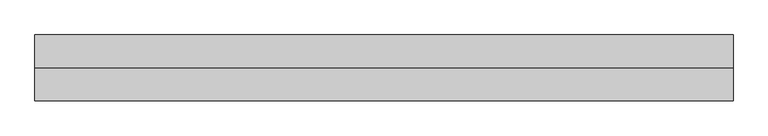
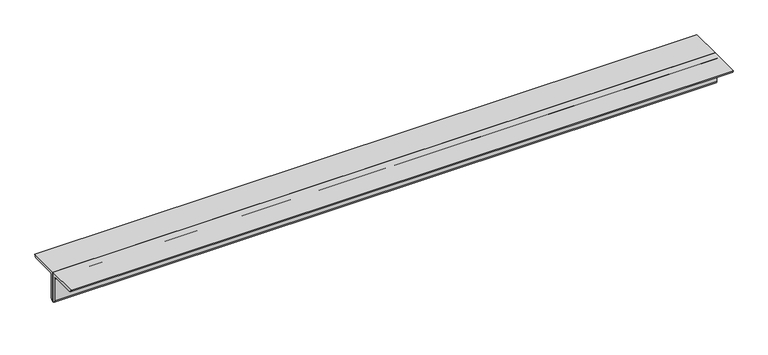
"""IFC4 building model written with IfcOpenShell, lengths in millimetres: member geometry, 0123_Steel Framing_2Ls-KSD3502 : H_SB_AR_S04_2Ls-130x130x12_VBR1."""

from ifc_helpers import new_model, si_unit, point, frame, frame_2d, origin, place, context, project, spatial, polyline, circle_curve, trimmed, segment, composite_curve, outline, extrude, source, transform, mapped, element, save


def member_630e65bb(model_context):
    return source(origin(), model_context, "Body", "SweptSolid", [
        extrude(outline(composite_curve([segment(polyline([(0.0, 36.4), (130.0, 36.4)]), True, "CONTINUOUS"), segment(trimmed(circle_curve(frame_2d((118.0, 36.4)), 12.0), [point((130.0, 36.4))], [point((118.0, 24.4))], False, "CARTESIAN"), True, "CONTINUOUS"), segment(polyline([(118.0, 24.4), (24.0, 24.4)]), True, "CONTINUOUS"), segment(trimmed(circle_curve(frame_2d((24.0, 12.4)), 12.0), [point((24.0, 24.4))], [point((12.0, 12.4))], True, "CARTESIAN"), True, "CONTINUOUS"), segment(polyline([(12.0, 12.4), (12.0, -81.6)]), True, "CONTINUOUS"), segment(trimmed(circle_curve(frame_2d((0.0, -81.6)), 12.0), [point((12.0, -81.6))], [point((0.0, -93.6))], False, "CARTESIAN"), True, "CONTINUOUS"), segment(polyline([(0.0, -93.6), (0.0, 36.4)]), True, "CONTINUOUS")], self_intersect=False)), frame((-1375.4177251, 0.0, 0.0), z_axis=(1.0, 0.0, 0.0), x_axis=(0.0, 1.0, 0.0)), (0.0, 0.0, 1.0), 2750.8354501),
        extrude(outline(composite_curve([segment(polyline([(0.0, 36.4), (0.0, -93.6)]), True, "CONTINUOUS"), segment(trimmed(circle_curve(frame_2d((0.0, -81.6)), 12.0), [point((0.0, -93.6))], [point((-12.0, -81.6))], False, "CARTESIAN"), True, "CONTINUOUS"), segment(polyline([(-12.0, -81.6), (-12.0, 12.4)]), True, "CONTINUOUS"), segment(trimmed(circle_curve(frame_2d((-24.0, 12.4)), 12.0), [point((-12.0, 12.4))], [point((-24.0, 24.4))], True, "CARTESIAN"), True, "CONTINUOUS"), segment(polyline([(-24.0, 24.4), (-118.0, 24.4)]), True, "CONTINUOUS"), segment(trimmed(circle_curve(frame_2d((-118.0, 36.4)), 12.0), [point((-118.0, 24.4))], [point((-130.0, 36.4))], False, "CARTESIAN"), True, "CONTINUOUS"), segment(polyline([(-130.0, 36.4), (0.0, 36.4)]), True, "CONTINUOUS")], self_intersect=False)), frame((-1375.4177251, 0.0, 0.0), z_axis=(1.0, 0.0, 0.0), x_axis=(0.0, 1.0, 0.0)), (0.0, 0.0, 1.0), 2750.8354501),
    ])


if __name__ == "__main__":
    model = new_model("IFC4")
    model_context = context("Model", 3, world=origin())
    ifc_project = project(units=[si_unit("LENGTHUNIT", "METRE", prefix="MILLI")], contexts=[model_context])
    site = spatial("IfcSite", under=ifc_project)
    building = spatial("IfcBuilding", under=site)
    placement = place(None, origin())
    member_shape = member_630e65bb(model_context)
    element("IfcMember", 1, ObjectType="0123_Steel Framing_2Ls-KSD3502 : H_SB_AR_S04_2Ls-130x130x12_VBR1", at=placement, inside=building, context=model_context, shape_type="MappedRepresentation", body=[
        mapped(member_shape, transform((0.0, 0.0, 0.0), x_axis=(1.0, 0.0, 0.0), y_axis=(0.0, 1.0, 0.0), z_axis=(0.0, 0.0, 1.0))),
    ])
    save(model, "model.ifc")

# Revit data of these elements
# Type "0123_Steel Framing_2Ls-KSD3502 : H_SB_AR_S04_2Ls-130x130x12_VBR1"
#   Assembly Code = "B10"
#   Legs = "SLBB"
#   W = 8.97
#   Perimeter = 1.04 m²/m
#   Nominal Weight = 46.80 kgf/m
#   Length [instance default] = 1000 mm
#   Space = 0 mm
#   b = 130 mm
#   d = 130 mm
#   t = 12 mm
#   y = 36.4 mm
#   A = 0.005952 m²
#   Structural Material [instance default] = Steel ASTM A36
# Element 1 (IfcMember, "0123_Steel Framing_2Ls-KSD3502 : H_SB_AR_S04_2Ls-130x130x12_VBR1")
#   Structural Material = Steel, 45-345
#   Materials on its faces: "Steel, 45-345"
# Materials
#   "Steel ASTM A36": class "Metal", colour RGB 199 199 199, transparency 0, Description = "Structural steel, ASTM A36 Grade B, mill finish", Cost = 0
#   "Steel, 45-345": class "Metal", colour RGB 189 187 185, transparency 0, Description = "Steel 345 MPa", Cost = 0
